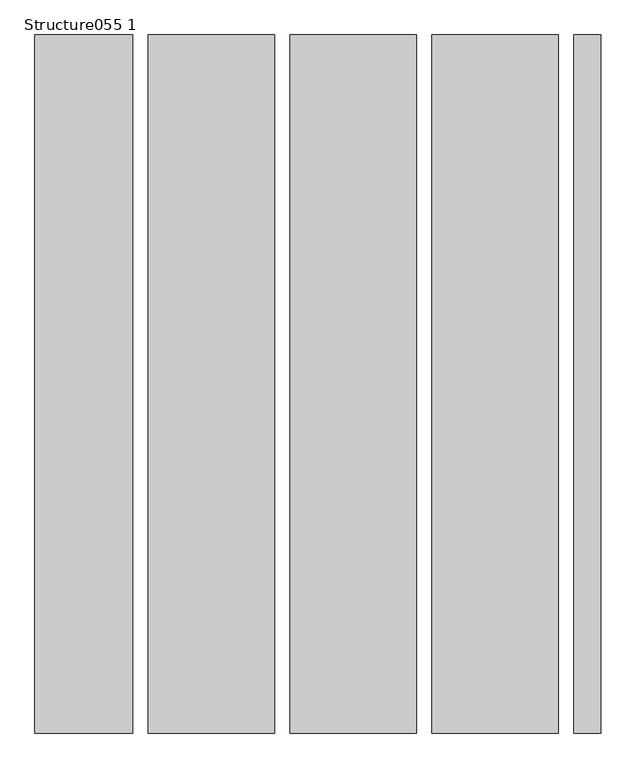
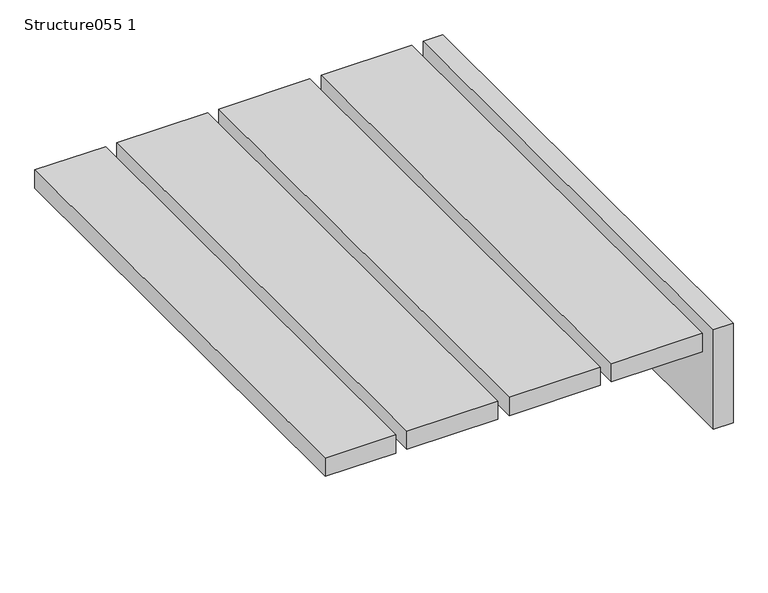
"""IFC4 building model written with IfcOpenShell, lengths in millimetres: proxy geometry, Structure055 1 : Structure055 10633."""

from ifc_helpers import new_model, si_unit, frame, origin, place, context, project, spatial, polyline, outline, extrude, source, transform, mapped, element, save


def structure055_1_aaac334e(model_context):
    return source(origin(), model_context, "Body", "SweptSolid", [
        extrude(outline(polyline([(6006.3637308, -1052.891), (5928.2662053, -1052.891), (5928.2662053, 947.109), (6006.3637308, 947.109), (6006.3637308, -1052.891)])), frame((0.0, 0.0, 42133.8036708), z_axis=(0.0, 0.0, 1.0), x_axis=(1.0, 0.0, 0.0)), (0.0, 0.0, 1.0), 418.8115316),
        extrude(outline(polyline([(5883.8162053, -1052.891), (5521.8662053, -1052.891), (5521.8662053, 947.109), (5883.8162053, 947.109), (5883.8162053, -1052.891)])), frame((0.0, 0.0, 42476.4152023), z_axis=(0.0, 0.0, 1.0), x_axis=(1.0, 0.0, 0.0)), (0.0, 0.0, 1.0), 76.2),
        extrude(outline(polyline([(4664.6162053, -1052.891), (4383.8162053, -1052.891), (4383.8162053, 947.109), (4664.6162053, 947.109), (4664.6162053, -1052.891)])), frame((0.0, 0.0, 42476.4152023), z_axis=(0.0, 0.0, 1.0), x_axis=(1.0, 0.0, 0.0)), (0.0, 0.0, 1.0), 76.2),
        extrude(outline(polyline([(5071.0162053, -1052.891), (4709.0662053, -1052.891), (4709.0662053, 947.109), (5071.0162053, 947.109), (5071.0162053, -1052.891)])), frame((0.0, 0.0, 42476.4152023), z_axis=(0.0, 0.0, 1.0), x_axis=(1.0, 0.0, 0.0)), (0.0, 0.0, 1.0), 76.2),
        extrude(outline(polyline([(5477.4162053, -1052.891), (5115.4662053, -1052.891), (5115.4662053, 947.109), (5477.4162053, 947.109), (5477.4162053, -1052.891)])), frame((0.0, 0.0, 42476.4152023), z_axis=(0.0, 0.0, 1.0), x_axis=(1.0, 0.0, 0.0)), (0.0, 0.0, 1.0), 76.2),
    ])


if __name__ == "__main__":
    model = new_model("IFC4")
    model_context = context("Model", 3, world=origin())
    ifc_project = project(units=[si_unit("LENGTHUNIT", "METRE", prefix="MILLI")], contexts=[model_context])
    site = spatial("IfcSite", under=ifc_project)
    building = spatial("IfcBuilding", under=site)
    placement = place(None, origin())
    structure055_1_shape = structure055_1_aaac334e(model_context)
    element("IfcBuildingElementProxy", 1, Name="Structure055 1 : Structure055 10633", ObjectType="Structure055 1 : Structure055 10633", at=placement, inside=building, context=model_context, shape_type="MappedRepresentation", body=[
        mapped(structure055_1_shape, transform((0.0, 0.0, 0.0), x_axis=(1.0, 0.0, 0.0), y_axis=(0.0, 1.0, 0.0), z_axis=(0.0, 0.0, 1.0))),
    ])
    save(model, "model.ifc")

# Revit data of these elements
# Type "Structure055 1 : Structure055 10633"
#   NameOverride = "Structure055"
# Element 1 (IfcBuildingElementProxy, "Structure055 1 : Structure055 10633")
#   Materials on its faces: "POLYURETHANE SPRAY FOAM UNDER ROOF SUBSTRATE (SEE T-24 ENERGY REPORT FOR R-VALUE)"
# Materials
#   "POLYURETHANE SPRAY FOAM UNDER ROOF SUBSTRATE (SEE T-24 ENERGY REPORT FOR R-VALUE)": class "Unassigned", colour RGB 210 164 194, transparency 0, Cost = 0
